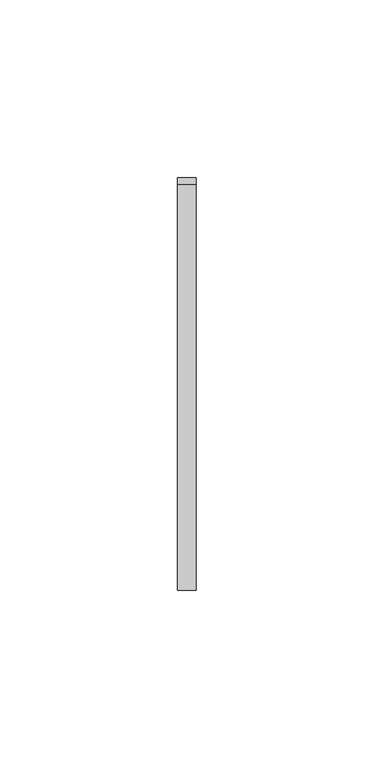
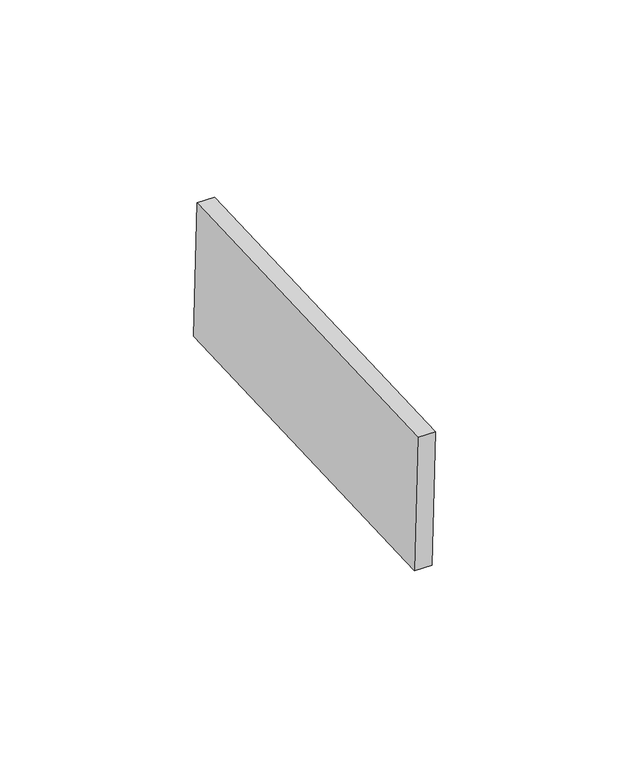
"""IFC4 building model written with IfcOpenShell, lengths in millimetres: proxy geometry, Inner panel:Inner panel:1:Inner panel:1 : Inner panel:Inner panel:300324:2:Inner panel:1:Inner panel:1 : Inner panel:Inner panel:300324:2 : Inner panel:Inner panel:1:Inner panel:1 : Inner panel:Inner panel:300324:300043:85 : Inner panel:Inner panel:1:Inner panel:1 : Inner panel:Inner panel:300324:2:Inner panel:1:Inner panel:1 : Inner panel:Inner panel:300324:2 : Inner panel:Inner panel:1:Inner panel:1 : Inner panel:Inner panel:300324:300043:308120."""

import ifcopenshell
import ifcopenshell.guid

model = None  # the IFC model being written
_history = None  # IfcOwnerHistory: only IFC2X3 demands one
_inside = {}  # id of a spatial element -> (the spatial element, [elements in it])
_under = {}  # id of a project, library or spatial element -> (it, [spatial elements below it])
_declared = {}  # id of a project -> (the project, [libraries it declares])
_typed = {}  # id of a type object -> (the type object, [elements of that type])
_made_of = {}  # id of a material, layer set ... -> (it, [elements and type objects made of it])


def new_model(schema):
    """Start an empty IFC model of exactly this schema.

    Asked for "IFC4X3", IfcOpenShell would pick the latest addendum, in which some entities
    have other attributes; the version numbers below select the first issue.
    IFC2X3 requires an IfcOwnerHistory on every rooted entity: one is made here for all.
    """
    global model, _history
    if schema == "IFC4X3":
        model = ifcopenshell.file(schema_version=(4, 3, 0, 0))
    else:
        model = ifcopenshell.file(schema=schema)
    _inside.clear()
    _under.clear()
    _declared.clear()
    _typed.clear()
    _made_of.clear()
    _history = None
    if model.schema == "IFC2X3":
        org = make("IfcOrganization", Name="unknown")
        user = make(
            "IfcPersonAndOrganization",
            ThePerson=make("IfcPerson", FamilyName="unknown"),
            TheOrganization=org,
        )
        app = make(
            "IfcApplication",
            ApplicationDeveloper=org,
            Version="unknown",
            ApplicationFullName="unknown",
            ApplicationIdentifier="unknown",
        )
        _history = make(
            "IfcOwnerHistory",
            OwningUser=user,
            OwningApplication=app,
            ChangeAction="ADDED",
            CreationDate=0,
        )
    return model


def make(cls, **values):
    """One entity of the class cls with the attributes given. An attribute that is None is left unset."""
    return model.create_entity(
        cls, **{name: value for name, value in values.items() if value is not None}
    )


def rooted(cls, **values):
    """An entity with a GlobalId (a new one), such as an element, a storey or a relation."""
    return make(cls, GlobalId=ifcopenshell.guid.new(), OwnerHistory=_history, **values)


def si_unit(unit_type, name, prefix=None):
    """IfcSIUnit, for example si_unit("LENGTHUNIT", "METRE", prefix="MILLI")."""
    return make("IfcSIUnit", UnitType=unit_type, Prefix=prefix, Name=name)


def assignment(units):
    """IfcUnitAssignment: the units of a project."""
    return None if units is None else make("IfcUnitAssignment", Units=units)


def point(xyz):
    """IfcCartesianPoint."""
    return None if xyz is None else make("IfcCartesianPoint", Coordinates=xyz)


def direction(xyz):
    """IfcDirection."""
    return None if xyz is None else make("IfcDirection", DirectionRatios=xyz)


def frame(location, z_axis=None, x_axis=None):
    """IfcAxis2Placement3D, a coordinate frame: its origin and axes. An axis left out is left unset."""
    return make(
        "IfcAxis2Placement3D",
        Location=point(location),
        Axis=direction(z_axis),
        RefDirection=direction(x_axis),
    )


def origin():
    """The frame at (0, 0, 0) with its axes left unset."""
    return frame((0.0, 0.0, 0.0))


def place(relative_to, where):
    """IfcLocalPlacement: puts the frame where relative to a parent placement (None: the world)."""
    return make(
        "IfcLocalPlacement", PlacementRelTo=relative_to, RelativePlacement=where
    )


def context(
    kind, dimensions, precision=None, world=None, true_north=None, identifier=None
):
    """IfcGeometricRepresentationContext, for example the 3D "Model" context."""
    return make(
        "IfcGeometricRepresentationContext",
        ContextIdentifier=identifier,
        ContextType=kind,
        CoordinateSpaceDimension=dimensions,
        Precision=precision,
        WorldCoordinateSystem=world,
        TrueNorth=true_north,
    )


def project(units=None, contexts=None):
    """IfcProject with its units and contexts."""
    return rooted(
        "IfcProject",
        Name="project",
        RepresentationContexts=contexts,
        UnitsInContext=assignment(units),
    )


def spatial(cls, under=None, at=None, **own):
    """A site, building, storey or space (cls), placed at a placement, below another one or the project."""
    s = rooted(cls, ObjectPlacement=at, **own)
    if under is not None:
        _under.setdefault(under.id(), (under, []))[1].append(s)
    return s


def polyline(points):
    """IfcPolyline through the points."""
    return make("IfcPolyline", Points=[point(p) for p in points])


def outline(outer, holes=None, kind="AREA"):
    """IfcArbitraryClosedProfileDef: a profile drawn as a closed curve; with holes, ...WithVoids."""
    if holes is None:
        return make("IfcArbitraryClosedProfileDef", ProfileType=kind, OuterCurve=outer)
    return make(
        "IfcArbitraryProfileDefWithVoids",
        ProfileType=kind,
        OuterCurve=outer,
        InnerCurves=holes,
    )


def extrude(swept, where, along, depth):
    """IfcExtrudedAreaSolid: the profile swept, set in the frame where, extruded along a direction by depth."""
    return make(
        "IfcExtrudedAreaSolid",
        SweptArea=swept,
        Position=where,
        ExtrudedDirection=direction(along),
        Depth=depth,
    )


def shape(context_of_items, identifier, shape_type, items):
    """IfcShapeRepresentation: the items that make up one representation, for example the "Body"."""
    return make(
        "IfcShapeRepresentation",
        ContextOfItems=context_of_items,
        RepresentationIdentifier=identifier,
        RepresentationType=shape_type,
        Items=items,
    )


def source(mapping_origin, context_of_items, identifier, shape_type, items):
    """IfcRepresentationMap: a shape defined once, which mapped items show again and again."""
    return make(
        "IfcRepresentationMap",
        MappingOrigin=mapping_origin,
        MappedRepresentation=shape(context_of_items, identifier, shape_type, items),
    )


def transform(
    local_origin,
    x_axis=None,
    y_axis=None,
    z_axis=None,
    scale=None,
    scale2=None,
    scale3=None,
    uniform=True,
):
    """IfcCartesianTransformationOperator3D, or its non-uniform kind. x_axis, y_axis, z_axis: its Axis1, 2, 3."""
    if uniform:
        return make(
            "IfcCartesianTransformationOperator3D",
            Axis1=direction(x_axis),
            Axis2=direction(y_axis),
            LocalOrigin=point(local_origin),
            Scale=scale,
            Axis3=direction(z_axis),
        )
    return make(
        "IfcCartesianTransformationOperator3DnonUniform",
        Axis1=direction(x_axis),
        Axis2=direction(y_axis),
        LocalOrigin=point(local_origin),
        Scale=scale,
        Axis3=direction(z_axis),
        Scale2=scale2,
        Scale3=scale3,
    )


def mapped(mapping_source, mapping_target):
    """IfcMappedItem: shows the shape of a source again, moved by a transform."""
    return make(
        "IfcMappedItem", MappingSource=mapping_source, MappingTarget=mapping_target
    )


def made_of(thing, what):
    """Note that an element or type object is made of a material, layer set ...; save() writes the relation."""
    if what is not None:
        _made_of.setdefault(what.id(), (what, []))[1].append(thing)
    return thing


def element(
    cls,
    number,
    at=None,
    inside=None,
    cuts=None,
    type_object=None,
    material=None,
    context=None,
    identifier="Body",
    shape_type=None,
    held_by="IfcProductDefinitionShape",
    body=None,
    shapes=None,
    **own,
):
    """One element of the class cls, such as IfcWall. Its Tag is "e" and its number.

    at: its placement. inside: the storey or other place that contains it. cuts: it is an
    opening in that element (IfcRelVoidsElement). A single representation is given by context,
    identifier, shape_type and body (its items); several are given by shapes. held_by: the class
    of the entity that holds the representations. save() writes the other relations.
    """
    e = rooted(cls, Tag="e%d" % number, ObjectPlacement=at, **own)
    if body is not None:
        shapes = [shape(context, identifier, shape_type, body)]
    if shapes is not None:
        e.Representation = make(held_by, Representations=shapes)
    if inside is not None:
        _inside.setdefault(inside.id(), (inside, []))[1].append(e)
    if cuts is not None:
        rooted(
            "IfcRelVoidsElement", RelatingBuildingElement=cuts, RelatedOpeningElement=e
        )
    if type_object is not None:
        _typed.setdefault(type_object.id(), (type_object, []))[1].append(e)
    return made_of(e, material)


def aggregate(whole, parts):
    """IfcRelAggregates: a whole, such as a stair, and the parts it consists of."""
    return rooted("IfcRelAggregates", RelatingObject=whole, RelatedObjects=parts)


def save(model, path):
    """Write the relations noted so far, then the file.

    IfcRelAggregates (storeys below a building ...), IfcRelContainedInSpatialStructure (elements
    in a storey), IfcRelDefinesByType, IfcRelAssociatesMaterial and IfcRelDeclares: one each for
    every whole, place, type object, material and project.
    """
    for whole, parts in _under.values():
        aggregate(whole, parts)
    for where, things in _inside.values():
        rooted(
            "IfcRelContainedInSpatialStructure",
            RelatedElements=things,
            RelatingStructure=where,
        )
    for kind, things in _typed.values():
        rooted("IfcRelDefinesByType", RelatedObjects=things, RelatingType=kind)
    for what, things in _made_of.values():
        rooted("IfcRelAssociatesMaterial", RelatedObjects=things, RelatingMaterial=what)
    for by, libraries in _declared.values():
        rooted("IfcRelDeclares", RelatingContext=by, RelatedDefinitions=libraries)
    model.write(path)


def generic_models_f186b848(model_context):
    return source(origin(), model_context, "Body", "SweptSolid", [
        extrude(outline(polyline([(0.0, -114.2999999), (0.0, 0.0), (5.2138089, 0.0), (5.2138089, -114.2999999), (0.0, -114.2999999)])), frame((592717.395117, -576618.8219505, 4051.6214343), z_axis=(0.0, -0.04163054471216399, 0.9991330730923527), x_axis=(-1.0, 0.0, 0.0)), (0.0, 0.0, 1.0), 43.2233908),
    ])


if __name__ == "__main__":
    model = new_model("IFC4")
    model_context = context("Model", 3, world=origin())
    ifc_project = project(units=[si_unit("LENGTHUNIT", "METRE", prefix="MILLI")], contexts=[model_context])
    site = spatial("IfcSite", under=ifc_project)
    building = spatial("IfcBuilding", under=site)
    placement = place(None, origin())
    generic_models_shape = generic_models_f186b848(model_context)
    element("IfcBuildingElementProxy", 1, Name="Inner panel:Inner panel:1:Inner panel:1 : Inner panel:Inner panel:300324:2:Inner panel:1:Inner panel:1 : Inner panel:Inner panel:300324:2 : Inner panel:Inner panel:1:Inner panel:1 : Inner panel:Inner panel:300324:300043:85 : Inner panel:Inner panel:1:Inner panel:1 : Inner panel:Inner panel:300324:2:Inner panel:1:Inner panel:1 : Inner panel:Inner panel:300324:2 : Inner panel:Inner panel:1:Inner panel:1 : Inner panel:Inner panel:300324:300043:308120", ObjectType="Inner panel:Inner panel:1:Inner panel:1 : Inner panel:Inner panel:300324:2:Inner panel:1:Inner panel:1 : Inner panel:Inner panel:300324:2 : Inner panel:Inner panel:1:Inner panel:1 : Inner panel:Inner panel:300324:300043:85 : Inner panel:Inner panel:1:Inner panel:1 : Inner panel:Inner panel:300324:2:Inner panel:1:Inner panel:1 : Inner panel:Inner panel:300324:2 : Inner panel:Inner panel:1:Inner panel:1 : Inner panel:Inner panel:300324:300043:308120", at=placement, inside=building, context=model_context, shape_type="MappedRepresentation", body=[
        mapped(generic_models_shape, transform((0.0, 0.0, 0.0), x_axis=(1.0, 0.0, 0.0), y_axis=(0.0, 1.0, 0.0), z_axis=(0.0, 0.0, 1.0))),
    ])
    save(model, "model.ifc")

# Revit data of these elements
# Type "Inner panel:Inner panel:1:Inner panel:1 : Inner panel:Inner panel:300324:2:Inner panel:1:Inner panel:1 : Inner panel:Inner panel:300324:2 : Inner panel:Inner panel:1:Inner panel:1 : Inner panel:Inner panel:300324:300043:85 : Inner panel:Inner panel:1:Inner panel:1 : Inner panel:Inner panel:300324:2:Inner panel:1:Inner panel:1 : Inner panel:Inner panel:300324:2 : Inner panel:Inner panel:1:Inner panel:1 : Inner panel:Inner panel:300324:300043:308120"
#   NameOverride = "Inner panel:Inner panel:1:Inner panel:1 : Inner panel:Inner panel:300324:2:Inner panel:1:Inner panel:1 : Inner panel:Inner panel:300324:2 : Inner panel:Inner panel:1:Inner panel:1 : Inner panel:Inner panel:300324:300043:308120"
#   ObjectTypeOverride = "Inner panel:1:Inner panel:1 : Inner panel:Inner panel:300324:2 : Inner panel:Inner panel:1:Inner panel:1 : Inner panel:Inner panel:300324:300043"
#   Reference = "Inner panel"
#   Tag = "308120"
# Element 1 (IfcBuildingElementProxy, "Inner panel:Inner panel:1:Inner panel:1 : Inner panel:Inner panel:300324:2:Inner panel:1:Inner panel:1 : Inner panel:Inner panel:300324:2 : Inner panel:Inner panel:1:Inner panel:1 : Inner panel:Inner panel:300324:300043:85 : Inner panel:Inner panel:1:Inner panel:1 : Inner panel:Inner panel:300324:2:Inner panel:1:Inner panel:1 : Inner panel:Inner panel:300324:2 : Inner panel:Inner panel:1:Inner panel:1 : Inner panel:Inner panel:300324:300043:308120")
#   Materials on its faces: "SLIDING CLIP"
# Materials
#   "SLIDING CLIP": class "Generic", colour RGB 120 120 120, transparency 0, Cost = 0
